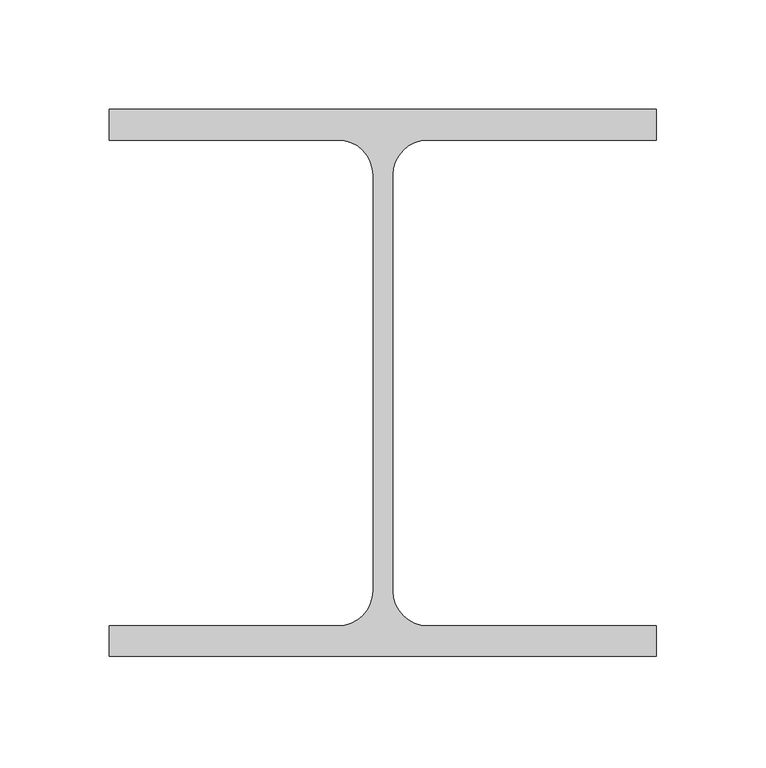
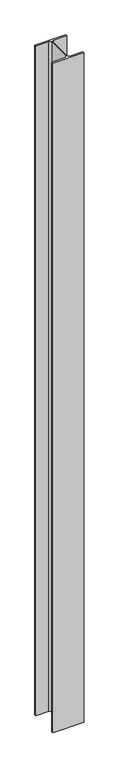
"""IFC4 building model written with IfcOpenShell, lengths in millimetres: column geometry, Steel Column_H_KSD3502 : H_SC_ASC_H-250x250x9x14."""

import ifcopenshell
import ifcopenshell.guid

model = None  # the IFC model being written
_history = None  # IfcOwnerHistory: only IFC2X3 demands one
_inside = {}  # id of a spatial element -> (the spatial element, [elements in it])
_under = {}  # id of a project, library or spatial element -> (it, [spatial elements below it])
_declared = {}  # id of a project -> (the project, [libraries it declares])
_typed = {}  # id of a type object -> (the type object, [elements of that type])
_made_of = {}  # id of a material, layer set ... -> (it, [elements and type objects made of it])


def new_model(schema):
    """Start an empty IFC model of exactly this schema.

    Asked for "IFC4X3", IfcOpenShell would pick the latest addendum, in which some entities
    have other attributes; the version numbers below select the first issue.
    IFC2X3 requires an IfcOwnerHistory on every rooted entity: one is made here for all.
    """
    global model, _history
    if schema == "IFC4X3":
        model = ifcopenshell.file(schema_version=(4, 3, 0, 0))
    else:
        model = ifcopenshell.file(schema=schema)
    _inside.clear()
    _under.clear()
    _declared.clear()
    _typed.clear()
    _made_of.clear()
    _history = None
    if model.schema == "IFC2X3":
        org = make("IfcOrganization", Name="unknown")
        user = make(
            "IfcPersonAndOrganization",
            ThePerson=make("IfcPerson", FamilyName="unknown"),
            TheOrganization=org,
        )
        app = make(
            "IfcApplication",
            ApplicationDeveloper=org,
            Version="unknown",
            ApplicationFullName="unknown",
            ApplicationIdentifier="unknown",
        )
        _history = make(
            "IfcOwnerHistory",
            OwningUser=user,
            OwningApplication=app,
            ChangeAction="ADDED",
            CreationDate=0,
        )
    return model


def make(cls, **values):
    """One entity of the class cls with the attributes given. An attribute that is None is left unset."""
    return model.create_entity(
        cls, **{name: value for name, value in values.items() if value is not None}
    )


def rooted(cls, **values):
    """An entity with a GlobalId (a new one), such as an element, a storey or a relation."""
    return make(cls, GlobalId=ifcopenshell.guid.new(), OwnerHistory=_history, **values)


def si_unit(unit_type, name, prefix=None):
    """IfcSIUnit, for example si_unit("LENGTHUNIT", "METRE", prefix="MILLI")."""
    return make("IfcSIUnit", UnitType=unit_type, Prefix=prefix, Name=name)


def assignment(units):
    """IfcUnitAssignment: the units of a project."""
    return None if units is None else make("IfcUnitAssignment", Units=units)


def point(xyz):
    """IfcCartesianPoint."""
    return None if xyz is None else make("IfcCartesianPoint", Coordinates=xyz)


def direction(xyz):
    """IfcDirection."""
    return None if xyz is None else make("IfcDirection", DirectionRatios=xyz)


def frame(location, z_axis=None, x_axis=None):
    """IfcAxis2Placement3D, a coordinate frame: its origin and axes. An axis left out is left unset."""
    return make(
        "IfcAxis2Placement3D",
        Location=point(location),
        Axis=direction(z_axis),
        RefDirection=direction(x_axis),
    )


def frame_2d(location, x_axis=None):
    """IfcAxis2Placement2D, a coordinate frame in the plane: its origin and x axis."""
    return make(
        "IfcAxis2Placement2D", Location=point(location), RefDirection=direction(x_axis)
    )


def origin():
    """The frame at (0, 0, 0) with its axes left unset."""
    return frame((0.0, 0.0, 0.0))


def place(relative_to, where):
    """IfcLocalPlacement: puts the frame where relative to a parent placement (None: the world)."""
    return make(
        "IfcLocalPlacement", PlacementRelTo=relative_to, RelativePlacement=where
    )


def context(
    kind, dimensions, precision=None, world=None, true_north=None, identifier=None
):
    """IfcGeometricRepresentationContext, for example the 3D "Model" context."""
    return make(
        "IfcGeometricRepresentationContext",
        ContextIdentifier=identifier,
        ContextType=kind,
        CoordinateSpaceDimension=dimensions,
        Precision=precision,
        WorldCoordinateSystem=world,
        TrueNorth=true_north,
    )


def project(units=None, contexts=None):
    """IfcProject with its units and contexts."""
    return rooted(
        "IfcProject",
        Name="project",
        RepresentationContexts=contexts,
        UnitsInContext=assignment(units),
    )


def spatial(cls, under=None, at=None, **own):
    """A site, building, storey or space (cls), placed at a placement, below another one or the project."""
    s = rooted(cls, ObjectPlacement=at, **own)
    if under is not None:
        _under.setdefault(under.id(), (under, []))[1].append(s)
    return s


def polyline(points):
    """IfcPolyline through the points."""
    return make("IfcPolyline", Points=[point(p) for p in points])


def circle_curve(where, radius):
    """IfcCircle in the frame where."""
    return make("IfcCircle", Position=where, Radius=radius)


def trimmed(basis, trim1, trim2, sense, master):
    """IfcTrimmedCurve: the piece of a basis curve between two trims."""
    return make(
        "IfcTrimmedCurve",
        BasisCurve=basis,
        Trim1=trim1,
        Trim2=trim2,
        SenseAgreement=sense,
        MasterRepresentation=master,
    )


def segment(curve, same_sense, transition):
    """IfcCompositeCurveSegment."""
    return make(
        "IfcCompositeCurveSegment",
        Transition=transition,
        SameSense=same_sense,
        ParentCurve=curve,
    )


def composite_curve(segments, self_intersect=None):
    """IfcCompositeCurve: segments joined end to end."""
    return make("IfcCompositeCurve", Segments=segments, SelfIntersect=self_intersect)


def outline(outer, holes=None, kind="AREA"):
    """IfcArbitraryClosedProfileDef: a profile drawn as a closed curve; with holes, ...WithVoids."""
    if holes is None:
        return make("IfcArbitraryClosedProfileDef", ProfileType=kind, OuterCurve=outer)
    return make(
        "IfcArbitraryProfileDefWithVoids",
        ProfileType=kind,
        OuterCurve=outer,
        InnerCurves=holes,
    )


def extrude(swept, where, along, depth):
    """IfcExtrudedAreaSolid: the profile swept, set in the frame where, extruded along a direction by depth."""
    return make(
        "IfcExtrudedAreaSolid",
        SweptArea=swept,
        Position=where,
        ExtrudedDirection=direction(along),
        Depth=depth,
    )


def shape(context_of_items, identifier, shape_type, items):
    """IfcShapeRepresentation: the items that make up one representation, for example the "Body"."""
    return make(
        "IfcShapeRepresentation",
        ContextOfItems=context_of_items,
        RepresentationIdentifier=identifier,
        RepresentationType=shape_type,
        Items=items,
    )


def source(mapping_origin, context_of_items, identifier, shape_type, items):
    """IfcRepresentationMap: a shape defined once, which mapped items show again and again."""
    return make(
        "IfcRepresentationMap",
        MappingOrigin=mapping_origin,
        MappedRepresentation=shape(context_of_items, identifier, shape_type, items),
    )


def transform(
    local_origin,
    x_axis=None,
    y_axis=None,
    z_axis=None,
    scale=None,
    scale2=None,
    scale3=None,
    uniform=True,
):
    """IfcCartesianTransformationOperator3D, or its non-uniform kind. x_axis, y_axis, z_axis: its Axis1, 2, 3."""
    if uniform:
        return make(
            "IfcCartesianTransformationOperator3D",
            Axis1=direction(x_axis),
            Axis2=direction(y_axis),
            LocalOrigin=point(local_origin),
            Scale=scale,
            Axis3=direction(z_axis),
        )
    return make(
        "IfcCartesianTransformationOperator3DnonUniform",
        Axis1=direction(x_axis),
        Axis2=direction(y_axis),
        LocalOrigin=point(local_origin),
        Scale=scale,
        Axis3=direction(z_axis),
        Scale2=scale2,
        Scale3=scale3,
    )


def mapped(mapping_source, mapping_target):
    """IfcMappedItem: shows the shape of a source again, moved by a transform."""
    return make(
        "IfcMappedItem", MappingSource=mapping_source, MappingTarget=mapping_target
    )


def made_of(thing, what):
    """Note that an element or type object is made of a material, layer set ...; save() writes the relation."""
    if what is not None:
        _made_of.setdefault(what.id(), (what, []))[1].append(thing)
    return thing


def element(
    cls,
    number,
    at=None,
    inside=None,
    cuts=None,
    type_object=None,
    material=None,
    context=None,
    identifier="Body",
    shape_type=None,
    held_by="IfcProductDefinitionShape",
    body=None,
    shapes=None,
    **own,
):
    """One element of the class cls, such as IfcWall. Its Tag is "e" and its number.

    at: its placement. inside: the storey or other place that contains it. cuts: it is an
    opening in that element (IfcRelVoidsElement). A single representation is given by context,
    identifier, shape_type and body (its items); several are given by shapes. held_by: the class
    of the entity that holds the representations. save() writes the other relations.
    """
    e = rooted(cls, Tag="e%d" % number, ObjectPlacement=at, **own)
    if body is not None:
        shapes = [shape(context, identifier, shape_type, body)]
    if shapes is not None:
        e.Representation = make(held_by, Representations=shapes)
    if inside is not None:
        _inside.setdefault(inside.id(), (inside, []))[1].append(e)
    if cuts is not None:
        rooted(
            "IfcRelVoidsElement", RelatingBuildingElement=cuts, RelatedOpeningElement=e
        )
    if type_object is not None:
        _typed.setdefault(type_object.id(), (type_object, []))[1].append(e)
    return made_of(e, material)


def aggregate(whole, parts):
    """IfcRelAggregates: a whole, such as a stair, and the parts it consists of."""
    return rooted("IfcRelAggregates", RelatingObject=whole, RelatedObjects=parts)


def save(model, path):
    """Write the relations noted so far, then the file.

    IfcRelAggregates (storeys below a building ...), IfcRelContainedInSpatialStructure (elements
    in a storey), IfcRelDefinesByType, IfcRelAssociatesMaterial and IfcRelDeclares: one each for
    every whole, place, type object, material and project.
    """
    for whole, parts in _under.values():
        aggregate(whole, parts)
    for where, things in _inside.values():
        rooted(
            "IfcRelContainedInSpatialStructure",
            RelatedElements=things,
            RelatingStructure=where,
        )
    for kind, things in _typed.values():
        rooted("IfcRelDefinesByType", RelatedObjects=things, RelatingType=kind)
    for what, things in _made_of.values():
        rooted("IfcRelAssociatesMaterial", RelatedObjects=things, RelatingMaterial=what)
    for by, libraries in _declared.values():
        rooted("IfcRelDeclares", RelatingContext=by, RelatedDefinitions=libraries)
    model.write(path)


def column_6a202524(model_context):
    return source(origin(), model_context, "Body", "SweptSolid", [
        extrude(outline(composite_curve([segment(polyline([(125.0, 125.0), (125.0, 111.0), (20.5, 111.0)]), True, "CONTINUOUS"), segment(trimmed(circle_curve(frame_2d((20.5, 95.0)), 16.0), [point((20.5, 111.0))], [point((4.5, 95.0))], True, "CARTESIAN"), True, "CONTINUOUS"), segment(polyline([(4.5, 95.0), (4.5, -95.0)]), True, "CONTINUOUS"), segment(trimmed(circle_curve(frame_2d((20.5, -95.0)), 16.0), [point((4.5, -95.0))], [point((20.5, -111.0))], True, "CARTESIAN"), True, "CONTINUOUS"), segment(polyline([(20.5, -111.0), (125.0, -111.0), (125.0, -125.0), (-125.0, -125.0), (-125.0, -111.0), (-20.5, -111.0)]), True, "CONTINUOUS"), segment(trimmed(circle_curve(frame_2d((-20.5, -95.0)), 16.0), [point((-20.5, -111.0))], [point((-4.5, -95.0))], True, "CARTESIAN"), True, "CONTINUOUS"), segment(polyline([(-4.5, -95.0), (-4.5, 95.0)]), True, "CONTINUOUS"), segment(trimmed(circle_curve(frame_2d((-20.5, 95.0)), 16.0), [point((-4.5, 95.0))], [point((-20.5, 111.0))], True, "CARTESIAN"), True, "CONTINUOUS"), segment(polyline([(-20.5, 111.0), (-125.0, 111.0), (-125.0, 125.0), (125.0, 125.0)]), True, "CONTINUOUS")], self_intersect=False)), frame((0.0, 0.0, 599.9720055), z_axis=(0.0, 0.0, 1.0), x_axis=(1.0, 0.0, 0.0)), (0.0, 0.0, 1.0), 5700.0),
    ])


if __name__ == "__main__":
    model = new_model("IFC4")
    model_context = context("Model", 3, world=origin())
    ifc_project = project(units=[si_unit("LENGTHUNIT", "METRE", prefix="MILLI")], contexts=[model_context])
    site = spatial("IfcSite", under=ifc_project)
    building = spatial("IfcBuilding", under=site)
    placement = place(None, origin())
    column_shape = column_6a202524(model_context)
    element("IfcColumn", 1, ObjectType="Steel Column_H_KSD3502 : H_SC_ASC_H-250x250x9x14", at=placement, inside=building, context=model_context, shape_type="MappedRepresentation", body=[
        mapped(column_shape, transform((0.0, 0.0, 0.0), x_axis=(1.0, 0.0, 0.0), y_axis=(0.0, 1.0, 0.0), z_axis=(0.0, 0.0, 1.0))),
    ])
    save(model, "model.ifc")

# Revit data of these elements
# Type "Steel Column_H_KSD3502 : H_SC_ASC_H-250x250x9x14"
#   Width = 25.0 cm
#   Web Thickness = 0.9 cm
#   Web Fillet = 1.6 cm
#   Warping Constant = 507646.0 cm⁶
#   Torsional Moment of Inertia = 51.4681 cm⁴
#   Section Area = 92.18 cm²
#   Plastic Modulus weak axis = 444.0 cm³
#   Plastic Modulus strong axis = 960.0 cm³
#   Perimeter = 1.27 m²/m
#   Nominal Weight = 72.40 kgf/m
#   Moment of Inertia weak axis = 3650.00 cm⁴
#   Moment of Inertia strong axis = 10800.00 cm⁴
#   Height = 25.0 cm
#   Flange Thickness = 1.4 cm
#   Elastic Modulus weak axis = 292.0 cm³
#   Elastic Modulus strong axis = 867.0 cm³
#   Centroid Vertical = 12.5 cm
#   Centroid Horizontal = 12.5 cm
#   Bolt Spacing = 13.97 cm
#   Structural Material [instance default] = Steel, 45-345
#   Section Name Key = ""
#   Assembly Code = ""
# Element 1 (IfcColumn, "Steel Column_H_KSD3502 : H_SC_ASC_H-250x250x9x14")
#   Structural Material = A03AD029-00005_Anchor Bolt (Installation only)_M24
#   Materials on its faces: "A03AD029-00005_Anchor Bolt (Installation only)_M24"
# Materials
#   "Steel, 45-345": class "Metal", colour RGB 189 187 185, transparency 0, Description = "Steel 345 MPa", Cost = 0
#   "A03AD029-00005_Anchor Bolt (Installation only)_M24": class "Unassigned", colour RGB 84 83 81, transparency 0, Cost = 0
